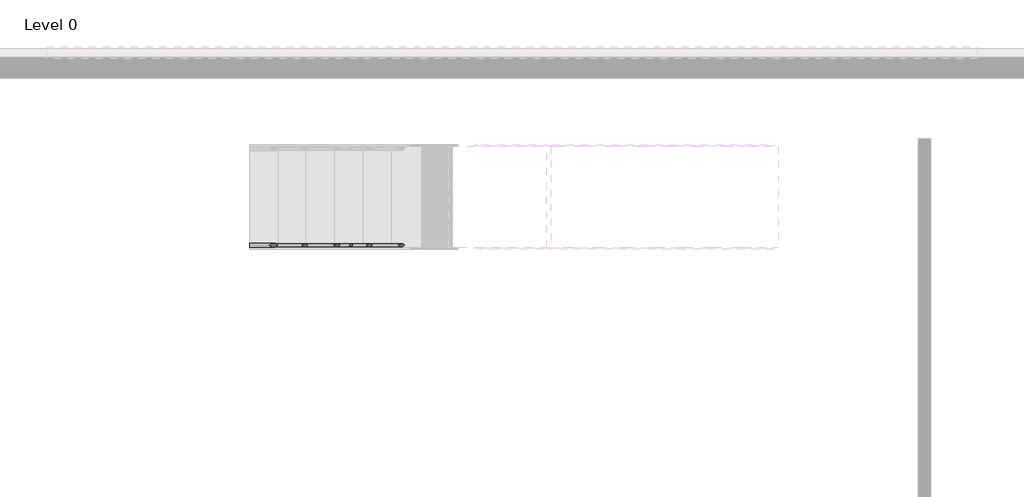
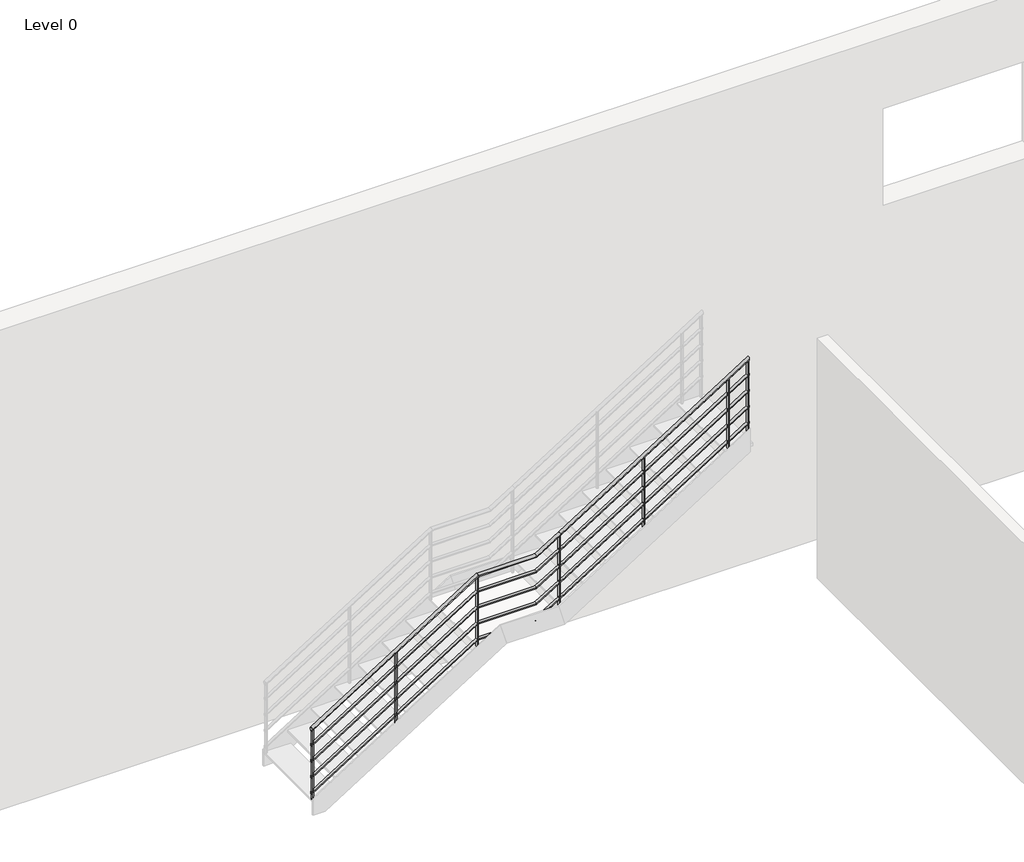
# One storey, part 2 of 3: 1 railing.
"""IFC4 building model written with IfcOpenShell, lengths in millimetres."""

from ifc_helpers import new_model, si_unit, frame, origin, place, context, project, spatial, circle_curve, ellipse_curve, element, save
from ifc_brep_helpers import plane_surface, cylinder_surface, advanced_brep

model = new_model("IFC4")

# Units and contexts
model_context = context("Model", 3, world=origin())
ifc_project = project(units=[si_unit("LENGTHUNIT", "METRE", prefix="MILLI")], contexts=[model_context])

# Site, building, storey
site = spatial("IfcSite", under=ifc_project)
building = spatial("IfcBuilding", under=site)
storey = spatial("IfcBuildingStorey", under=building, Name="Level 0", Elevation=0.0)

# Railing
placement = place(None, origin())
element("IfcRailing", 1, ObjectType="900mm_Pipe", at=placement, inside=storey, context=model_context, shape_type="AdvancedBrep", body=[
    advanced_brep(
    [(-5863.6361778, 8217.1063821, 1052.8297954), (-5863.6361778, 8257.1063821, 1052.8297954), (-694.2155657, 8217.1063821, 3876.3592072), (-694.2155657, 8257.1063821, 3876.3592072), (-3897.8594533, 8217.1063821, 2291.7647059), (-3897.8594533, 8257.1063821, 2291.7647059), (-3208.4388411, 8217.1063821, 2291.7647059), (-3208.4388411, 8257.1063821, 2291.7647059), (-2923.5517592, 8217.1063821, 2471.3153878), (-2923.5517592, 8257.1063821, 2471.3153878)],
    [
        (0, 1, ellipse_curve(frame((-5863.6361778, 8237.1063821, 1052.8297954), z_axis=(-1.0, 0.0, 0.0), x_axis=(0.0, 0.0, -1.0)), 23.6407928, 20.0)),
        (1, 0, ellipse_curve(frame((-5863.6361778, 8237.1063821, 1052.8297954), z_axis=(-1.0, 0.0, 0.0), x_axis=(0.0, 0.0, -1.0)), 23.6407928, 20.0)),
        (2, 3, ellipse_curve(frame((-694.2155657, 8237.1063821, 3876.3592072), z_axis=(1.0, 0.0, 0.0), x_axis=(0.0, 0.0, -1.0)), 23.6407928, 20.0)),
        (3, 2, ellipse_curve(frame((-694.2155657, 8237.1063821, 3876.3592072), z_axis=(1.0, 0.0, 0.0), x_axis=(0.0, 0.0, -1.0)), 23.6407928, 20.0)),
        (0, 4),
        (4, 5, ellipse_curve(frame((-3897.8594533, 8237.1063821, 2291.7647059), z_axis=(-0.9607276713561336, 0.0, -0.2774929575513964), x_axis=(0.2774929575513966, 0.0, -0.9607276713561334)), 20.8175538, 20.0)),
        (5, 1),
        (5, 4, ellipse_curve(frame((-3897.8594533, 8237.1063821, 2291.7647059), z_axis=(-0.9607276713561336, 0.0, -0.2774929575513964), x_axis=(0.2774929575513966, 0.0, -0.9607276713561334)), 20.8175538, 20.0)),
        (4, 6),
        (6, 7, ellipse_curve(frame((-3208.4388411, 8237.1063821, 2291.7647059), z_axis=(-0.9607276713561337, 0.0, -0.27749295755139625), x_axis=(-0.2774929575513956, 0.0, 0.9607276713561337)), 20.8175538, 20.0)),
        (7, 5),
        (7, 6, ellipse_curve(frame((-3208.4388411, 8237.1063821, 2291.7647059), z_axis=(-0.9607276713561337, 0.0, -0.27749295755139625), x_axis=(-0.2774929575513956, 0.0, 0.9607276713561337)), 20.8175538, 20.0)),
        (6, 8),
        (8, 9, circle_curve(frame((-2923.5517592, 8237.1063821, 2471.3153878), z_axis=(-0.8459953170187583, 0.0, -0.5331903258521585), x_axis=(0.0, 1.0, 0.0)), 20.0)),
        (9, 7),
        (9, 8, circle_curve(frame((-2923.5517592, 8237.1063821, 2471.3153878), z_axis=(-0.8459953170187583, 0.0, -0.5331903258521585), x_axis=(0.0, 1.0, 0.0)), 20.0)),
        (8, 2),
        (3, 9),
    ],
    [
        plane_surface(frame((-5863.6361778, 8237.1063821, 1076.4705882), z_axis=(-1.0, 0.0, 0.0), x_axis=(0.0, 1.0, 0.0))),
        plane_surface(frame((-694.2155657, 8237.1063821, 3900.0), z_axis=(1.0, 0.0, 0.0), x_axis=(0.0, 1.0, 0.0))),
        cylinder_surface(frame((-5852.9723713, 8237.1063821, 1059.5506819), z_axis=(-0.8459953170187579, 0.0, -0.5331903258521589), x_axis=(0.0, 1.0, 0.0)), 20.0),
        cylinder_surface(frame((-3903.6361778, 8237.1063821, 2291.7647059), z_axis=(-1.0, 0.0, 0.0), x_axis=(0.0, 1.0, 0.0)), 20.0),
        cylinder_surface(frame((-3203.5517592, 8237.1063821, 2294.8447995), z_axis=(-0.8459953170187581, 0.0, -0.5331903258521584), x_axis=(0.0, 1.0, 0.0)), 20.0),
        cylinder_surface(frame((-2923.5517592, 8237.1063821, 2471.3153878), z_axis=(-0.8459953170187582, 0.0, -0.5331903258521583), x_axis=(0.0, 1.0, 0.0)), 20.0),
    ],
    [
        (0, [[1, 2]]),
        (1, [[3, 4]]),
        (2, [[-1, 5, 6, 7]]),
        (2, [[-2, -7, 8, -5]]),
        (3, [[-6, 9, 10, 11]]),
        (3, [[-8, -11, 12, -9]]),
        (4, [[-10, 13, 14, 15]]),
        (4, [[-12, -15, 16, -13]]),
        (5, [[-14, 17, -4, 18]]),
        (5, [[-16, -18, -3, -17]]),
    ],
),
    advanced_brep(
    [(-5863.6361778, 8252.1063821, 858.7399936), (-5863.6361778, 8222.1063821, 858.7399936), (-3903.6361778, 8252.1063821, 2094.0341113), (-3903.6361778, 8222.1063821, 2094.0341113)],
    [
        (0, 1, ellipse_curve(frame((-5863.6361778, 8237.1063821, 858.7399936), z_axis=(-1.0, 0.0, 0.0), x_axis=(0.0, 0.0, -1.0)), 17.7305946, 15.0)),
        (1, 0, ellipse_curve(frame((-5863.6361778, 8237.1063821, 858.7399936), z_axis=(-1.0, 0.0, 0.0), x_axis=(0.0, 0.0, -1.0)), 17.7305946, 15.0)),
        (2, 3, ellipse_curve(frame((-3903.6361778, 8237.1063821, 2094.0341113), z_axis=(1.0, 0.0, 0.0), x_axis=(0.0, 0.0, -1.0)), 17.7305946, 15.0)),
        (3, 2, ellipse_curve(frame((-3903.6361778, 8237.1063821, 2094.0341113), z_axis=(1.0, 0.0, 0.0), x_axis=(0.0, 0.0, -1.0)), 17.7305946, 15.0)),
        (0, 2),
        (3, 1),
    ],
    [
        plane_surface(frame((-5863.6361778, 8237.1063821, 876.4705882), z_axis=(-1.0, 0.0, 0.0), x_axis=(0.0, 1.0, 0.0))),
        plane_surface(frame((-3903.6361778, 8237.1063821, 2111.7647059), z_axis=(1.0, 0.0, 0.0), x_axis=(0.0, 1.0, 0.0))),
        cylinder_surface(frame((-5855.6383229, 8237.1063821, 863.7806585), z_axis=(-0.8459953170187579, 0.0, -0.5331903258521589), x_axis=(0.0, -1.0, 0.0)), 15.0),
    ],
    [
        (0, [[1, 2]]),
        (1, [[3, 4]]),
        (2, [[-1, 5, -4, 6]]),
        (2, [[-2, -6, -3, -5]]),
    ],
),
    advanced_brep(
    [(-3903.6361778, 8252.1063821, 2096.7647059), (-3903.6361778, 8222.1063821, 2096.7647059), (-3209.8830223, 8252.1063821, 2096.7647059), (-3209.8830223, 8222.1063821, 2096.7647059), (-2934.2155657, 8252.1063821, 2270.5046995), (-2934.2155657, 8222.1063821, 2270.5046995)],
    [
        (0, 1, circle_curve(frame((-3903.6361778, 8237.1063821, 2096.7647059), z_axis=(-1.0, 0.0, 0.0), x_axis=(0.0, -1.0, 0.0)), 15.0)),
        (1, 0, circle_curve(frame((-3903.6361778, 8237.1063821, 2096.7647059), z_axis=(-1.0, 0.0, 0.0), x_axis=(0.0, -1.0, 0.0)), 15.0)),
        (0, 2),
        (2, 3, ellipse_curve(frame((-3209.8830223, 8237.1063821, 2096.7647059), z_axis=(-0.9607276713561337, 0.0, -0.27749295755139614), x_axis=(-0.27749295755139564, 0.0, 0.9607276713561337)), 15.6131654, 15.0)),
        (3, 1),
        (3, 2, ellipse_curve(frame((-3209.8830223, 8237.1063821, 2096.7647059), z_axis=(-0.9607276713561337, 0.0, -0.27749295755139614), x_axis=(-0.27749295755139564, 0.0, 0.9607276713561337)), 15.6131654, 15.0)),
        (4, 5, ellipse_curve(frame((-2934.2155657, 8237.1063821, 2270.5046995), z_axis=(1.0, 0.0, 0.0), x_axis=(0.0, 0.0, -1.0)), 17.7305946, 15.0)),
        (5, 4, ellipse_curve(frame((-2934.2155657, 8237.1063821, 2270.5046995), z_axis=(1.0, 0.0, 0.0), x_axis=(0.0, 0.0, -1.0)), 17.7305946, 15.0)),
        (2, 4),
        (5, 3),
    ],
    [
        plane_surface(frame((-3903.6361778, 8237.1063821, 2111.7647059), z_axis=(-1.0, 0.0, 0.0), x_axis=(0.0, 1.0, 0.0))),
        cylinder_surface(frame((-3903.6361778, 8237.1063821, 2096.7647059), z_axis=(-1.0, 0.0, 0.0), x_axis=(0.0, -1.0, 0.0)), 15.0),
        plane_surface(frame((-2934.2155657, 8237.1063821, 2288.2352941), z_axis=(1.0, 0.0, 0.0), x_axis=(0.0, 1.0, 0.0))),
        cylinder_surface(frame((-3206.2177108, 8237.1063821, 2099.0747761), z_axis=(-0.8459953170187581, 0.0, -0.5331903258521584), x_axis=(0.0, -1.0, 0.0)), 15.0),
    ],
    [
        (0, [[1, 2]]),
        (1, [[-1, 3, 4, 5]]),
        (1, [[-2, -5, 6, -3]]),
        (2, [[7, 8]]),
        (3, [[-4, 9, -8, 10]]),
        (3, [[-6, -10, -7, -9]]),
    ],
),
    advanced_brep(
    [(-2934.2155657, 8252.1063821, 2270.5046995), (-2934.2155657, 8222.1063821, 2270.5046995), (-694.2155657, 8252.1063821, 3682.2694054), (-694.2155657, 8222.1063821, 3682.2694054)],
    [
        (0, 1, ellipse_curve(frame((-2934.2155657, 8237.1063821, 2270.5046995), z_axis=(-1.0, 0.0, 0.0), x_axis=(0.0, 0.0, -1.0)), 17.7305946, 15.0)),
        (1, 0, ellipse_curve(frame((-2934.2155657, 8237.1063821, 2270.5046995), z_axis=(-1.0, 0.0, 0.0), x_axis=(0.0, 0.0, -1.0)), 17.7305946, 15.0)),
        (2, 3, ellipse_curve(frame((-694.2155657, 8237.1063821, 3682.2694054), z_axis=(1.0, 0.0, 0.0), x_axis=(0.0, 0.0, -1.0)), 17.7305946, 15.0)),
        (3, 2, ellipse_curve(frame((-694.2155657, 8237.1063821, 3682.2694054), z_axis=(1.0, 0.0, 0.0), x_axis=(0.0, 0.0, -1.0)), 17.7305946, 15.0)),
        (0, 2),
        (3, 1),
    ],
    [
        plane_surface(frame((-2934.2155657, 8237.1063821, 2288.2352941), z_axis=(-1.0, 0.0, 0.0), x_axis=(0.0, 1.0, 0.0))),
        plane_surface(frame((-694.2155657, 8237.1063821, 3700.0), z_axis=(1.0, 0.0, 0.0), x_axis=(0.0, 1.0, 0.0))),
        cylinder_surface(frame((-2926.2177108, 8237.1063821, 2275.5453644), z_axis=(-0.8459953170187582, 0.0, -0.5331903258521584), x_axis=(0.0, -1.0, 0.0)), 15.0),
    ],
    [
        (0, [[1, 2]]),
        (1, [[3, 4]]),
        (2, [[-1, 5, -4, 6]]),
        (2, [[-2, -6, -3, -5]]),
    ],
),
    advanced_brep(
    [(-5863.6361778, 8252.1063821, 658.7399936), (-5863.6361778, 8222.1063821, 658.7399936), (-3903.6361778, 8252.1063821, 1894.0341113), (-3903.6361778, 8222.1063821, 1894.0341113)],
    [
        (0, 1, ellipse_curve(frame((-5863.6361778, 8237.1063821, 658.7399936), z_axis=(-1.0, 0.0, 0.0), x_axis=(0.0, 0.0, -1.0)), 17.7305946, 15.0)),
        (1, 0, ellipse_curve(frame((-5863.6361778, 8237.1063821, 658.7399936), z_axis=(-1.0, 0.0, 0.0), x_axis=(0.0, 0.0, -1.0)), 17.7305946, 15.0)),
        (2, 3, ellipse_curve(frame((-3903.6361778, 8237.1063821, 1894.0341113), z_axis=(1.0, 0.0, 0.0), x_axis=(0.0, 0.0, -1.0)), 17.7305946, 15.0)),
        (3, 2, ellipse_curve(frame((-3903.6361778, 8237.1063821, 1894.0341113), z_axis=(1.0, 0.0, 0.0), x_axis=(0.0, 0.0, -1.0)), 17.7305946, 15.0)),
        (0, 2),
        (3, 1),
    ],
    [
        plane_surface(frame((-5863.6361778, 8237.1063821, 676.4705882), z_axis=(-1.0, 0.0, 0.0), x_axis=(0.0, 1.0, 0.0))),
        plane_surface(frame((-3903.6361778, 8237.1063821, 1911.7647059), z_axis=(1.0, 0.0, 0.0), x_axis=(0.0, 1.0, 0.0))),
        cylinder_surface(frame((-5855.6383229, 8237.1063821, 663.7806585), z_axis=(-0.8459953170187579, 0.0, -0.5331903258521589), x_axis=(0.0, -1.0, 0.0)), 15.0),
    ],
    [
        (0, [[1, 2]]),
        (1, [[3, 4]]),
        (2, [[-1, 5, -4, 6]]),
        (2, [[-2, -6, -3, -5]]),
    ],
),
    advanced_brep(
    [(-3903.6361778, 8252.1063821, 1896.7647059), (-3903.6361778, 8222.1063821, 1896.7647059), (-3209.8830223, 8252.1063821, 1896.7647059), (-3209.8830223, 8222.1063821, 1896.7647059), (-2934.2155657, 8252.1063821, 2070.5046995), (-2934.2155657, 8222.1063821, 2070.5046995)],
    [
        (0, 1, circle_curve(frame((-3903.6361778, 8237.1063821, 1896.7647059), z_axis=(-1.0, 0.0, 0.0), x_axis=(0.0, -1.0, 0.0)), 15.0)),
        (1, 0, circle_curve(frame((-3903.6361778, 8237.1063821, 1896.7647059), z_axis=(-1.0, 0.0, 0.0), x_axis=(0.0, -1.0, 0.0)), 15.0)),
        (0, 2),
        (2, 3, ellipse_curve(frame((-3209.8830223, 8237.1063821, 1896.7647059), z_axis=(-0.9607276713561337, 0.0, -0.27749295755139614), x_axis=(-0.27749295755139564, 0.0, 0.9607276713561337)), 15.6131654, 15.0)),
        (3, 1),
        (3, 2, ellipse_curve(frame((-3209.8830223, 8237.1063821, 1896.7647059), z_axis=(-0.9607276713561337, 0.0, -0.27749295755139614), x_axis=(-0.27749295755139564, 0.0, 0.9607276713561337)), 15.6131654, 15.0)),
        (4, 5, ellipse_curve(frame((-2934.2155657, 8237.1063821, 2070.5046995), z_axis=(1.0, 0.0, 0.0), x_axis=(0.0, 0.0, -1.0)), 17.7305946, 15.0)),
        (5, 4, ellipse_curve(frame((-2934.2155657, 8237.1063821, 2070.5046995), z_axis=(1.0, 0.0, 0.0), x_axis=(0.0, 0.0, -1.0)), 17.7305946, 15.0)),
        (2, 4),
        (5, 3),
    ],
    [
        plane_surface(frame((-3903.6361778, 8237.1063821, 1911.7647059), z_axis=(-1.0, 0.0, 0.0), x_axis=(0.0, 1.0, 0.0))),
        cylinder_surface(frame((-3903.6361778, 8237.1063821, 1896.7647059), z_axis=(-1.0, 0.0, 0.0), x_axis=(0.0, -1.0, 0.0)), 15.0),
        plane_surface(frame((-2934.2155657, 8237.1063821, 2088.2352941), z_axis=(1.0, 0.0, 0.0), x_axis=(0.0, 1.0, 0.0))),
        cylinder_surface(frame((-3206.2177108, 8237.1063821, 1899.0747761), z_axis=(-0.8459953170187581, 0.0, -0.5331903258521584), x_axis=(0.0, -1.0, 0.0)), 15.0),
    ],
    [
        (0, [[1, 2]]),
        (1, [[-1, 3, 4, 5]]),
        (1, [[-2, -5, 6, -3]]),
        (2, [[7, 8]]),
        (3, [[-4, 9, -8, 10]]),
        (3, [[-6, -10, -7, -9]]),
    ],
),
    advanced_brep(
    [(-2934.2155657, 8252.1063821, 2070.5046995), (-2934.2155657, 8222.1063821, 2070.5046995), (-694.2155657, 8252.1063821, 3482.2694054), (-694.2155657, 8222.1063821, 3482.2694054)],
    [
        (0, 1, ellipse_curve(frame((-2934.2155657, 8237.1063821, 2070.5046995), z_axis=(-1.0, 0.0, 0.0), x_axis=(0.0, 0.0, -1.0)), 17.7305946, 15.0)),
        (1, 0, ellipse_curve(frame((-2934.2155657, 8237.1063821, 2070.5046995), z_axis=(-1.0, 0.0, 0.0), x_axis=(0.0, 0.0, -1.0)), 17.7305946, 15.0)),
        (2, 3, ellipse_curve(frame((-694.2155657, 8237.1063821, 3482.2694054), z_axis=(1.0, 0.0, 0.0), x_axis=(0.0, 0.0, -1.0)), 17.7305946, 15.0)),
        (3, 2, ellipse_curve(frame((-694.2155657, 8237.1063821, 3482.2694054), z_axis=(1.0, 0.0, 0.0), x_axis=(0.0, 0.0, -1.0)), 17.7305946, 15.0)),
        (0, 2),
        (3, 1),
    ],
    [
        plane_surface(frame((-2934.2155657, 8237.1063821, 2088.2352941), z_axis=(-1.0, 0.0, 0.0), x_axis=(0.0, 1.0, 0.0))),
        plane_surface(frame((-694.2155657, 8237.1063821, 3500.0), z_axis=(1.0, 0.0, 0.0), x_axis=(0.0, 1.0, 0.0))),
        cylinder_surface(frame((-2926.2177108, 8237.1063821, 2075.5453644), z_axis=(-0.8459953170187582, 0.0, -0.5331903258521584), x_axis=(0.0, -1.0, 0.0)), 15.0),
    ],
    [
        (0, [[1, 2]]),
        (1, [[3, 4]]),
        (2, [[-1, 5, -4, 6]]),
        (2, [[-2, -6, -3, -5]]),
    ],
),
    advanced_brep(
    [(-5863.6361778, 8252.1063821, 458.7399936), (-5863.6361778, 8222.1063821, 458.7399936), (-3903.6361778, 8252.1063821, 1694.0341113), (-3903.6361778, 8222.1063821, 1694.0341113)],
    [
        (0, 1, ellipse_curve(frame((-5863.6361778, 8237.1063821, 458.7399936), z_axis=(-1.0, 0.0, 0.0), x_axis=(0.0, 0.0, -1.0)), 17.7305946, 15.0)),
        (1, 0, ellipse_curve(frame((-5863.6361778, 8237.1063821, 458.7399936), z_axis=(-1.0, 0.0, 0.0), x_axis=(0.0, 0.0, -1.0)), 17.7305946, 15.0)),
        (2, 3, ellipse_curve(frame((-3903.6361778, 8237.1063821, 1694.0341113), z_axis=(1.0, 0.0, 0.0), x_axis=(0.0, 0.0, -1.0)), 17.7305946, 15.0)),
        (3, 2, ellipse_curve(frame((-3903.6361778, 8237.1063821, 1694.0341113), z_axis=(1.0, 0.0, 0.0), x_axis=(0.0, 0.0, -1.0)), 17.7305946, 15.0)),
        (0, 2),
        (3, 1),
    ],
    [
        plane_surface(frame((-5863.6361778, 8237.1063821, 476.4705882), z_axis=(-1.0, 0.0, 0.0), x_axis=(0.0, 1.0, 0.0))),
        plane_surface(frame((-3903.6361778, 8237.1063821, 1711.7647059), z_axis=(1.0, 0.0, 0.0), x_axis=(0.0, 1.0, 0.0))),
        cylinder_surface(frame((-5855.6383229, 8237.1063821, 463.7806585), z_axis=(-0.8459953170187579, 0.0, -0.5331903258521589), x_axis=(0.0, -1.0, 0.0)), 15.0),
    ],
    [
        (0, [[1, 2]]),
        (1, [[3, 4]]),
        (2, [[-1, 5, -4, 6]]),
        (2, [[-2, -6, -3, -5]]),
    ],
),
    advanced_brep(
    [(-3903.6361778, 8252.1063821, 1696.7647059), (-3903.6361778, 8222.1063821, 1696.7647059), (-3209.8830223, 8252.1063821, 1696.7647059), (-3209.8830223, 8222.1063821, 1696.7647059), (-2934.2155657, 8252.1063821, 1870.5046995), (-2934.2155657, 8222.1063821, 1870.5046995)],
    [
        (0, 1, circle_curve(frame((-3903.6361778, 8237.1063821, 1696.7647059), z_axis=(-1.0, 0.0, 0.0), x_axis=(0.0, -1.0, 0.0)), 15.0)),
        (1, 0, circle_curve(frame((-3903.6361778, 8237.1063821, 1696.7647059), z_axis=(-1.0, 0.0, 0.0), x_axis=(0.0, -1.0, 0.0)), 15.0)),
        (0, 2),
        (2, 3, ellipse_curve(frame((-3209.8830223, 8237.1063821, 1696.7647059), z_axis=(-0.9607276713561337, 0.0, -0.27749295755139614), x_axis=(-0.27749295755139564, 0.0, 0.9607276713561337)), 15.6131654, 15.0)),
        (3, 1),
        (3, 2, ellipse_curve(frame((-3209.8830223, 8237.1063821, 1696.7647059), z_axis=(-0.9607276713561337, 0.0, -0.27749295755139614), x_axis=(-0.27749295755139564, 0.0, 0.9607276713561337)), 15.6131654, 15.0)),
        (4, 5, ellipse_curve(frame((-2934.2155657, 8237.1063821, 1870.5046995), z_axis=(1.0, 0.0, 0.0), x_axis=(0.0, 0.0, -1.0)), 17.7305946, 15.0)),
        (5, 4, ellipse_curve(frame((-2934.2155657, 8237.1063821, 1870.5046995), z_axis=(1.0, 0.0, 0.0), x_axis=(0.0, 0.0, -1.0)), 17.7305946, 15.0)),
        (2, 4),
        (5, 3),
    ],
    [
        plane_surface(frame((-3903.6361778, 8237.1063821, 1711.7647059), z_axis=(-1.0, 0.0, 0.0), x_axis=(0.0, 1.0, 0.0))),
        cylinder_surface(frame((-3903.6361778, 8237.1063821, 1696.7647059), z_axis=(-1.0, 0.0, 0.0), x_axis=(0.0, -1.0, 0.0)), 15.0),
        plane_surface(frame((-2934.2155657, 8237.1063821, 1888.2352941), z_axis=(1.0, 0.0, 0.0), x_axis=(0.0, 1.0, 0.0))),
        cylinder_surface(frame((-3206.2177108, 8237.1063821, 1699.0747761), z_axis=(-0.8459953170187581, 0.0, -0.5331903258521584), x_axis=(0.0, -1.0, 0.0)), 15.0),
    ],
    [
        (0, [[1, 2]]),
        (1, [[-1, 3, 4, 5]]),
        (1, [[-2, -5, 6, -3]]),
        (2, [[7, 8]]),
        (3, [[-4, 9, -8, 10]]),
        (3, [[-6, -10, -7, -9]]),
    ],
),
    advanced_brep(
    [(-2934.2155657, 8252.1063821, 1870.5046995), (-2934.2155657, 8222.1063821, 1870.5046995), (-694.2155657, 8252.1063821, 3282.2694054), (-694.2155657, 8222.1063821, 3282.2694054)],
    [
        (0, 1, ellipse_curve(frame((-2934.2155657, 8237.1063821, 1870.5046995), z_axis=(-1.0, 0.0, 0.0), x_axis=(0.0, 0.0, -1.0)), 17.7305946, 15.0)),
        (1, 0, ellipse_curve(frame((-2934.2155657, 8237.1063821, 1870.5046995), z_axis=(-1.0, 0.0, 0.0), x_axis=(0.0, 0.0, -1.0)), 17.7305946, 15.0)),
        (2, 3, ellipse_curve(frame((-694.2155657, 8237.1063821, 3282.2694054), z_axis=(1.0, 0.0, 0.0), x_axis=(0.0, 0.0, -1.0)), 17.7305946, 15.0)),
        (3, 2, ellipse_curve(frame((-694.2155657, 8237.1063821, 3282.2694054), z_axis=(1.0, 0.0, 0.0), x_axis=(0.0, 0.0, -1.0)), 17.7305946, 15.0)),
        (0, 2),
        (3, 1),
    ],
    [
        plane_surface(frame((-2934.2155657, 8237.1063821, 1888.2352941), z_axis=(-1.0, 0.0, 0.0), x_axis=(0.0, 1.0, 0.0))),
        plane_surface(frame((-694.2155657, 8237.1063821, 3300.0), z_axis=(1.0, 0.0, 0.0), x_axis=(0.0, 1.0, 0.0))),
        cylinder_surface(frame((-2926.2177108, 8237.1063821, 1875.5453644), z_axis=(-0.8459953170187582, 0.0, -0.5331903258521584), x_axis=(0.0, -1.0, 0.0)), 15.0),
    ],
    [
        (0, [[1, 2]]),
        (1, [[3, 4]]),
        (2, [[-1, 5, -4, 6]]),
        (2, [[-2, -6, -3, -5]]),
    ],
),
    advanced_brep(
    [(-5863.6361778, 8252.1063821, 258.7399936), (-5863.6361778, 8222.1063821, 258.7399936), (-3903.6361778, 8252.1063821, 1494.0341113), (-3903.6361778, 8222.1063821, 1494.0341113)],
    [
        (0, 1, ellipse_curve(frame((-5863.6361778, 8237.1063821, 258.7399936), z_axis=(-1.0, 0.0, 0.0), x_axis=(0.0, 0.0, -1.0)), 17.7305946, 15.0)),
        (1, 0, ellipse_curve(frame((-5863.6361778, 8237.1063821, 258.7399936), z_axis=(-1.0, 0.0, 0.0), x_axis=(0.0, 0.0, -1.0)), 17.7305946, 15.0)),
        (2, 3, ellipse_curve(frame((-3903.6361778, 8237.1063821, 1494.0341113), z_axis=(1.0, 0.0, 0.0), x_axis=(0.0, 0.0, -1.0)), 17.7305946, 15.0)),
        (3, 2, ellipse_curve(frame((-3903.6361778, 8237.1063821, 1494.0341113), z_axis=(1.0, 0.0, 0.0), x_axis=(0.0, 0.0, -1.0)), 17.7305946, 15.0)),
        (0, 2),
        (3, 1),
    ],
    [
        plane_surface(frame((-5863.6361778, 8237.1063821, 276.4705882), z_axis=(-1.0, 0.0, 0.0), x_axis=(0.0, 1.0, 0.0))),
        plane_surface(frame((-3903.6361778, 8237.1063821, 1511.7647059), z_axis=(1.0, 0.0, 0.0), x_axis=(0.0, 1.0, 0.0))),
        cylinder_surface(frame((-5855.6383229, 8237.1063821, 263.7806585), z_axis=(-0.8459953170187579, 0.0, -0.5331903258521589), x_axis=(0.0, -1.0, 0.0)), 15.0),
    ],
    [
        (0, [[1, 2]]),
        (1, [[3, 4]]),
        (2, [[-1, 5, -4, 6]]),
        (2, [[-2, -6, -3, -5]]),
    ],
),
    advanced_brep(
    [(-3903.6361778, 8252.1063821, 1496.7647059), (-3903.6361778, 8222.1063821, 1496.7647059), (-3209.8830223, 8252.1063821, 1496.7647059), (-3209.8830223, 8222.1063821, 1496.7647059), (-2934.2155657, 8252.1063821, 1670.5046995), (-2934.2155657, 8222.1063821, 1670.5046995)],
    [
        (0, 1, circle_curve(frame((-3903.6361778, 8237.1063821, 1496.7647059), z_axis=(-1.0, 0.0, 0.0), x_axis=(0.0, -1.0, 0.0)), 15.0)),
        (1, 0, circle_curve(frame((-3903.6361778, 8237.1063821, 1496.7647059), z_axis=(-1.0, 0.0, 0.0), x_axis=(0.0, -1.0, 0.0)), 15.0)),
        (0, 2),
        (2, 3, ellipse_curve(frame((-3209.8830223, 8237.1063821, 1496.7647059), z_axis=(-0.9607276713561337, 0.0, -0.27749295755139614), x_axis=(-0.27749295755139564, 0.0, 0.9607276713561337)), 15.6131654, 15.0)),
        (3, 1),
        (3, 2, ellipse_curve(frame((-3209.8830223, 8237.1063821, 1496.7647059), z_axis=(-0.9607276713561337, 0.0, -0.27749295755139614), x_axis=(-0.27749295755139564, 0.0, 0.9607276713561337)), 15.6131654, 15.0)),
        (4, 5, ellipse_curve(frame((-2934.2155657, 8237.1063821, 1670.5046995), z_axis=(1.0, 0.0, 0.0), x_axis=(0.0, 0.0, -1.0)), 17.7305946, 15.0)),
        (5, 4, ellipse_curve(frame((-2934.2155657, 8237.1063821, 1670.5046995), z_axis=(1.0, 0.0, 0.0), x_axis=(0.0, 0.0, -1.0)), 17.7305946, 15.0)),
        (2, 4),
        (5, 3),
    ],
    [
        plane_surface(frame((-3903.6361778, 8237.1063821, 1511.7647059), z_axis=(-1.0, 0.0, 0.0), x_axis=(0.0, 1.0, 0.0))),
        cylinder_surface(frame((-3903.6361778, 8237.1063821, 1496.7647059), z_axis=(-1.0, 0.0, 0.0), x_axis=(0.0, -1.0, 0.0)), 15.0),
        plane_surface(frame((-2934.2155657, 8237.1063821, 1688.2352941), z_axis=(1.0, 0.0, 0.0), x_axis=(0.0, 1.0, 0.0))),
        cylinder_surface(frame((-3206.2177108, 8237.1063821, 1499.0747761), z_axis=(-0.8459953170187581, 0.0, -0.5331903258521584), x_axis=(0.0, -1.0, 0.0)), 15.0),
    ],
    [
        (0, [[1, 2]]),
        (1, [[-1, 3, 4, 5]]),
        (1, [[-2, -5, 6, -3]]),
        (2, [[7, 8]]),
        (3, [[-4, 9, -8, 10]]),
        (3, [[-6, -10, -7, -9]]),
    ],
),
    advanced_brep(
    [(-2934.2155657, 8252.1063821, 1670.5046995), (-2934.2155657, 8222.1063821, 1670.5046995), (-694.2155657, 8252.1063821, 3082.2694054), (-694.2155657, 8222.1063821, 3082.2694054)],
    [
        (0, 1, ellipse_curve(frame((-2934.2155657, 8237.1063821, 1670.5046995), z_axis=(-1.0, 0.0, 0.0), x_axis=(0.0, 0.0, -1.0)), 17.7305946, 15.0)),
        (1, 0, ellipse_curve(frame((-2934.2155657, 8237.1063821, 1670.5046995), z_axis=(-1.0, 0.0, 0.0), x_axis=(0.0, 0.0, -1.0)), 17.7305946, 15.0)),
        (2, 3, ellipse_curve(frame((-694.2155657, 8237.1063821, 3082.2694054), z_axis=(1.0, 0.0, 0.0), x_axis=(0.0, 0.0, -1.0)), 17.7305946, 15.0)),
        (3, 2, ellipse_curve(frame((-694.2155657, 8237.1063821, 3082.2694054), z_axis=(1.0, 0.0, 0.0), x_axis=(0.0, 0.0, -1.0)), 17.7305946, 15.0)),
        (0, 2),
        (3, 1),
    ],
    [
        plane_surface(frame((-2934.2155657, 8237.1063821, 1688.2352941), z_axis=(-1.0, 0.0, 0.0), x_axis=(0.0, 1.0, 0.0))),
        plane_surface(frame((-694.2155657, 8237.1063821, 3100.0), z_axis=(1.0, 0.0, 0.0), x_axis=(0.0, 1.0, 0.0))),
        cylinder_surface(frame((-2926.2177108, 8237.1063821, 1675.5453644), z_axis=(-0.8459953170187582, 0.0, -0.5331903258521584), x_axis=(0.0, -1.0, 0.0)), 15.0),
    ],
    [
        (0, [[1, 2]]),
        (1, [[3, 4]]),
        (2, [[-1, 5, -4, 6]]),
        (2, [[-2, -6, -3, -5]]),
    ],
),
    advanced_brep(
    [(-934.2155657, 8224.6063821, 3701.4579102), (-934.2155657, 8224.6063821, 2823.5294118), (-934.2155657, 8249.6063821, 2823.5294118), (-934.2155657, 8249.6063821, 3701.4579102)],
    [
        (0, 1),
        (1, 2, circle_curve(frame((-934.2155657, 8237.1063821, 2823.5294118), z_axis=(0.0, 0.0, 1.0), x_axis=(0.0, 1.0, 0.0)), 12.5)),
        (2, 3),
        (3, 0, ellipse_curve(frame((-934.2155657, 8237.1063821, 3701.4579102), z_axis=(0.5331903258521581, 0.0, -0.8459953170187584), x_axis=(0.8459953170187585, 0.0, 0.533190325852158)), 14.7754955, 12.5)),
        (0, 3, ellipse_curve(frame((-934.2155657, 8237.1063821, 3701.4579102), z_axis=(0.5331903258521581, 0.0, -0.8459953170187584), x_axis=(0.8459953170187585, 0.0, 0.533190325852158)), 14.7754955, 12.5)),
        (2, 1, circle_curve(frame((-934.2155657, 8237.1063821, 2823.5294118), z_axis=(0.0, 0.0, 1.0), x_axis=(0.0, 1.0, 0.0)), 12.5)),
    ],
    [
        cylinder_surface(frame((-934.2155657, 8237.1063821, 2723.5294118), z_axis=(0.0, 0.0, 1.0), x_axis=(0.0, 1.0, 0.0)), 12.5),
        plane_surface(frame((-909.2155657, 8262.1063821, 3717.2142127), z_axis=(-0.5331903258521581, 0.0, 0.8459953170187584), x_axis=(0.0, -1.0, 0.0))),
        plane_surface(frame((-959.2155657, 8262.1063821, 2823.5294118), z_axis=(0.0, 0.0, -1.0), x_axis=(0.0, -1.0, 0.0))),
    ],
    [
        (0, [[1, 2, 3, 4]]),
        (0, [[-1, 5, -3, 6]]),
        (1, [[-4, -5]]),
        (2, [[-2, -6]]),
    ],
),
    advanced_brep(
    [(-1934.2155657, 8224.6063821, 3071.2058094), (-1934.2155657, 8224.6063821, 2117.6470588), (-1934.2155657, 8249.6063821, 2117.6470588), (-1934.2155657, 8249.6063821, 3071.2058094)],
    [
        (0, 1),
        (1, 2, circle_curve(frame((-1934.2155657, 8237.1063821, 2117.6470588), z_axis=(0.0, 0.0, 1.0), x_axis=(0.0, 1.0, 0.0)), 12.5)),
        (2, 3),
        (3, 0, ellipse_curve(frame((-1934.2155657, 8237.1063821, 3071.2058094), z_axis=(0.5331903258521581, 0.0, -0.8459953170187584), x_axis=(0.8459953170187585, 0.0, 0.533190325852158)), 14.7754955, 12.5)),
        (0, 3, ellipse_curve(frame((-1934.2155657, 8237.1063821, 3071.2058094), z_axis=(0.5331903258521581, 0.0, -0.8459953170187584), x_axis=(0.8459953170187585, 0.0, 0.533190325852158)), 14.7754955, 12.5)),
        (2, 1, circle_curve(frame((-1934.2155657, 8237.1063821, 2117.6470588), z_axis=(0.0, 0.0, 1.0), x_axis=(0.0, 1.0, 0.0)), 12.5)),
    ],
    [
        cylinder_surface(frame((-1934.2155657, 8237.1063821, 2017.6470588), z_axis=(0.0, 0.0, 1.0), x_axis=(0.0, 1.0, 0.0)), 12.5),
        plane_surface(frame((-1909.2155657, 8262.1063821, 3086.9621119), z_axis=(-0.5331903258521581, 0.0, 0.8459953170187584), x_axis=(0.0, -1.0, 0.0))),
        plane_surface(frame((-1959.2155657, 8262.1063821, 2117.6470588), z_axis=(0.0, 0.0, -1.0), x_axis=(0.0, -1.0, 0.0))),
    ],
    [
        (0, [[1, 2, 3, 4]]),
        (0, [[-1, 5, -3, 6]]),
        (1, [[-4, -5]]),
        (2, [[-2, -6]]),
    ],
),
    advanced_brep(
    [(-4863.6361778, 8224.6063821, 1659.4411035), (-4863.6361778, 8224.6063821, 705.8823529), (-4863.6361778, 8249.6063821, 705.8823529), (-4863.6361778, 8249.6063821, 1659.4411035)],
    [
        (0, 1),
        (1, 2, circle_curve(frame((-4863.6361778, 8237.1063821, 705.8823529), z_axis=(0.0, 0.0, 1.0), x_axis=(0.0, 1.0, 0.0)), 12.5)),
        (2, 3),
        (3, 0, ellipse_curve(frame((-4863.6361778, 8237.1063821, 1659.4411035), z_axis=(0.5331903258521581, 0.0, -0.8459953170187584), x_axis=(0.8459953170187585, 0.0, 0.533190325852158)), 14.7754955, 12.5)),
        (0, 3, ellipse_curve(frame((-4863.6361778, 8237.1063821, 1659.4411035), z_axis=(0.5331903258521581, 0.0, -0.8459953170187584), x_axis=(0.8459953170187585, 0.0, 0.533190325852158)), 14.7754955, 12.5)),
        (2, 1, circle_curve(frame((-4863.6361778, 8237.1063821, 705.8823529), z_axis=(0.0, 0.0, 1.0), x_axis=(0.0, 1.0, 0.0)), 12.5)),
    ],
    [
        cylinder_surface(frame((-4863.6361778, 8237.1063821, 605.8823529), z_axis=(0.0, 0.0, 1.0), x_axis=(0.0, 1.0, 0.0)), 12.5),
        plane_surface(frame((-4838.6361778, 8262.1063821, 1675.197406), z_axis=(-0.5331903258521581, 0.0, 0.8459953170187584), x_axis=(0.0, -1.0, 0.0))),
        plane_surface(frame((-4888.6361778, 8262.1063821, 705.8823529), z_axis=(0.0, 0.0, -1.0), x_axis=(0.0, -1.0, 0.0))),
    ],
    [
        (0, [[1, 2, 3, 4]]),
        (0, [[-1, 5, -3, 6]]),
        (1, [[-4, -5]]),
        (2, [[-2, -6]]),
    ],
),
    advanced_brep(
    [(-2934.2155657, 8224.6063821, 2440.9537085), (-2934.2155657, 8224.6063821, 1411.7647059), (-2934.2155657, 8249.6063821, 1411.7647059), (-2934.2155657, 8249.6063821, 2440.9537085)],
    [
        (0, 1),
        (1, 2, circle_curve(frame((-2934.2155657, 8237.1063821, 1411.7647059), z_axis=(0.0, 0.0, 1.0), x_axis=(0.0, 1.0, 0.0)), 12.5)),
        (2, 3),
        (3, 0, ellipse_curve(frame((-2934.2155657, 8237.1063821, 2440.9537085), z_axis=(0.5331903258521598, 0.0, -0.8459953170187574), x_axis=(0.8459953170187573, 0.0, 0.5331903258521594)), 14.7754955, 12.5)),
        (0, 3, ellipse_curve(frame((-2934.2155657, 8237.1063821, 2440.9537085), z_axis=(0.5331903258521598, 0.0, -0.8459953170187574), x_axis=(0.8459953170187573, 0.0, 0.5331903258521594)), 14.7754955, 12.5)),
        (2, 1, circle_curve(frame((-2934.2155657, 8237.1063821, 1411.7647059), z_axis=(0.0, 0.0, 1.0), x_axis=(0.0, 1.0, 0.0)), 12.5)),
    ],
    [
        cylinder_surface(frame((-2934.2155657, 8237.1063821, 1311.7647059), z_axis=(0.0, 0.0, 1.0), x_axis=(0.0, 1.0, 0.0)), 12.5),
        plane_surface(frame((-2909.2155657, 8262.1063821, 2456.710011), z_axis=(-0.5331903258521598, 0.0, 0.8459953170187574), x_axis=(0.0, -1.0, 0.0))),
        plane_surface(frame((-2959.2155657, 8262.1063821, 1411.7647059), z_axis=(0.0, 0.0, -1.0), x_axis=(0.0, -1.0, 0.0))),
    ],
    [
        (0, [[1, 2, 3, 4]]),
        (0, [[-1, 5, -3, 6]]),
        (1, [[-4, -5]]),
        (2, [[-2, -6]]),
    ],
),
    advanced_brep(
    [(-3903.6361778, 8224.6063821, 2264.4831203), (-3903.6361778, 8224.6063821, 1411.7647059), (-3903.6361778, 8249.6063821, 1411.7647059), (-3903.6361778, 8249.6063821, 2264.4831203)],
    [
        (0, 1),
        (1, 2, circle_curve(frame((-3903.6361778, 8237.1063821, 1411.7647059), z_axis=(0.0, 0.0, 1.0), x_axis=(0.0, 1.0, 0.0)), 12.5)),
        (2, 3),
        (3, 0, ellipse_curve(frame((-3903.6361778, 8237.1063821, 2264.4831203), z_axis=(0.5331903258521598, 0.0, -0.8459953170187574), x_axis=(0.8459953170187573, 0.0, 0.5331903258521594)), 14.7754955, 12.5)),
        (0, 3, ellipse_curve(frame((-3903.6361778, 8237.1063821, 2264.4831203), z_axis=(0.5331903258521598, 0.0, -0.8459953170187574), x_axis=(0.8459953170187573, 0.0, 0.5331903258521594)), 14.7754955, 12.5)),
        (2, 1, circle_curve(frame((-3903.6361778, 8237.1063821, 1411.7647059), z_axis=(0.0, 0.0, 1.0), x_axis=(0.0, 1.0, 0.0)), 12.5)),
    ],
    [
        cylinder_surface(frame((-3903.6361778, 8237.1063821, 1311.7647059), z_axis=(0.0, 0.0, 1.0), x_axis=(0.0, 1.0, 0.0)), 12.5),
        plane_surface(frame((-3878.6361778, 8262.1063821, 2280.2394228), z_axis=(-0.5331903258521598, 0.0, 0.8459953170187574), x_axis=(0.0, -1.0, 0.0))),
        plane_surface(frame((-3928.6361778, 8262.1063821, 1411.7647059), z_axis=(0.0, 0.0, -1.0), x_axis=(0.0, -1.0, 0.0))),
    ],
    [
        (0, [[1, 2, 3, 4]]),
        (0, [[-1, 5, -3, 6]]),
        (1, [[-4, -5]]),
        (2, [[-2, -6]]),
    ],
),
    advanced_brep(
    [(-706.7155657, 8224.6063821, 3844.8402631), (-706.7155657, 8224.6063821, 2823.5294118), (-706.7155657, 8249.6063821, 2823.5294118), (-706.7155657, 8249.6063821, 3844.8402631)],
    [
        (0, 1),
        (1, 2, circle_curve(frame((-706.7155657, 8237.1063821, 2823.5294118), z_axis=(0.0, 0.0, 1.0), x_axis=(0.0, 1.0, 0.0)), 12.5)),
        (2, 3),
        (3, 0, ellipse_curve(frame((-706.7155657, 8237.1063821, 3844.8402631), z_axis=(0.5331903258521581, 0.0, -0.8459953170187584), x_axis=(0.8459953170187585, 0.0, 0.533190325852158)), 14.7754955, 12.5)),
        (0, 3, ellipse_curve(frame((-706.7155657, 8237.1063821, 3844.8402631), z_axis=(0.5331903258521581, 0.0, -0.8459953170187584), x_axis=(0.8459953170187585, 0.0, 0.533190325852158)), 14.7754955, 12.5)),
        (2, 1, circle_curve(frame((-706.7155657, 8237.1063821, 2823.5294118), z_axis=(0.0, 0.0, 1.0), x_axis=(0.0, 1.0, 0.0)), 12.5)),
    ],
    [
        cylinder_surface(frame((-706.7155657, 8237.1063821, 2723.5294118), z_axis=(0.0, 0.0, 1.0), x_axis=(0.0, 1.0, 0.0)), 12.5),
        plane_surface(frame((-681.7155657, 8262.1063821, 3860.5965657), z_axis=(-0.5331903258521581, 0.0, 0.8459953170187584), x_axis=(0.0, -1.0, 0.0))),
        plane_surface(frame((-731.7155657, 8262.1063821, 2823.5294118), z_axis=(0.0, 0.0, -1.0), x_axis=(0.0, -1.0, 0.0))),
    ],
    [
        (0, [[1, 2, 3, 4]]),
        (0, [[-1, 5, -3, 6]]),
        (1, [[-4, -5]]),
        (2, [[-2, -6]]),
    ],
),
    advanced_brep(
    [(-5851.1361778, 8224.6063821, 1037.0671539), (-5851.1361778, 8224.6063821, 176.4705882), (-5851.1361778, 8249.6063821, 176.4705882), (-5851.1361778, 8249.6063821, 1037.0671539)],
    [
        (0, 1),
        (1, 2, circle_curve(frame((-5851.1361778, 8237.1063821, 176.4705882), z_axis=(0.0, 0.0, 1.0), x_axis=(0.0, 1.0, 0.0)), 12.5)),
        (2, 3),
        (3, 0, ellipse_curve(frame((-5851.1361778, 8237.1063821, 1037.0671539), z_axis=(0.5331903258521598, 0.0, -0.8459953170187574), x_axis=(0.8459953170187573, 0.0, 0.5331903258521594)), 14.7754955, 12.5)),
        (0, 3, ellipse_curve(frame((-5851.1361778, 8237.1063821, 1037.0671539), z_axis=(0.5331903258521598, 0.0, -0.8459953170187574), x_axis=(0.8459953170187573, 0.0, 0.5331903258521594)), 14.7754955, 12.5)),
        (2, 1, circle_curve(frame((-5851.1361778, 8237.1063821, 176.4705882), z_axis=(0.0, 0.0, 1.0), x_axis=(0.0, 1.0, 0.0)), 12.5)),
    ],
    [
        cylinder_surface(frame((-5851.1361778, 8237.1063821, 76.4705882), z_axis=(0.0, 0.0, 1.0), x_axis=(0.0, 1.0, 0.0)), 12.5),
        plane_surface(frame((-5826.1361778, 8262.1063821, 1052.8234564), z_axis=(-0.5331903258521598, 0.0, 0.8459953170187574), x_axis=(0.0, -1.0, 0.0))),
        plane_surface(frame((-5876.1361778, 8262.1063821, 176.4705882), z_axis=(0.0, 0.0, -1.0), x_axis=(0.0, -1.0, 0.0))),
    ],
    [
        (0, [[1, 2, 3, 4]]),
        (0, [[-1, 5, -3, 6]]),
        (1, [[-4, -5]]),
        (2, [[-2, -6]]),
    ],
),
])

save(model, "model.ifc")

# Revit data of these elements
# Type "900mm_Pipe"
#   built-in parameter 1008612 = 0.019685 (stored number, unit not read)
#   built-in parameter 1008611 = 0.0984252 (stored number, unit not read)
#   built-in parameter 1008609 = 3.28084 (stored number, unit not read)
#   built-in parameter 1008604 = 0.19685 (stored number, unit not read)
#   built-in parameter 1008603 = 0.164042 (stored number, unit not read)
#   Railing Height = 900 mm
#   built-in parameter 1008630 = 2
#   built-in parameter 1008610 = 1
#   built-in parameter 1008605 = 1
#   built-in parameter 1008618 = Baluster_Round : 25mm
# Element 1 (IfcRailing, "900mm_Pipe")
#   Phase Created = New Construction
